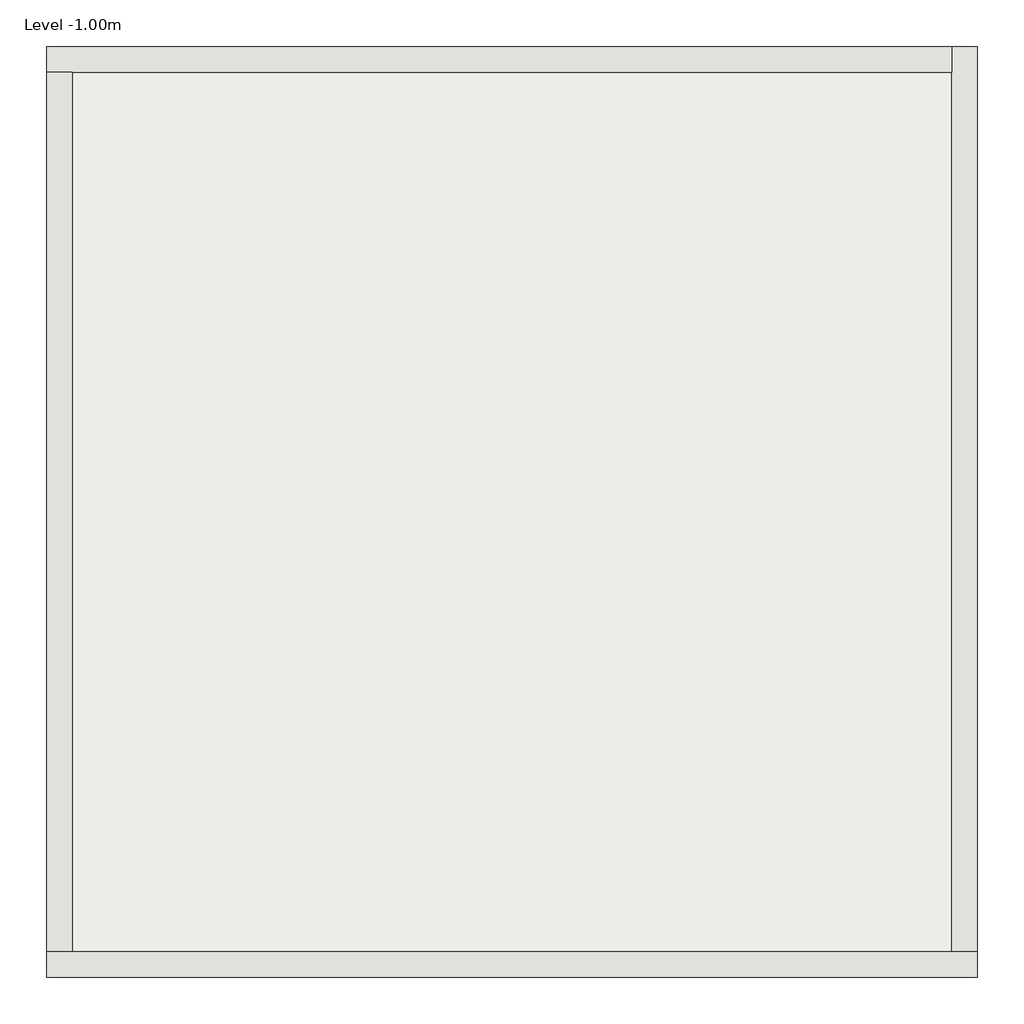
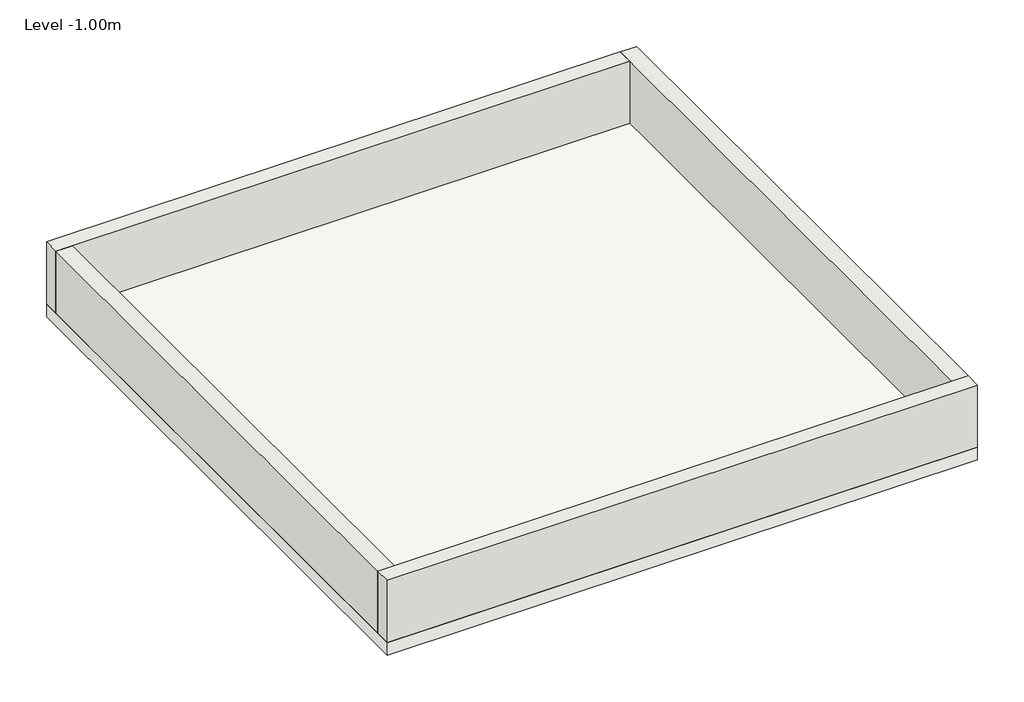
# One storey: 4 walls, 1 slab.
"""IFC4 building model written with IfcOpenShell, lengths in millimetres."""

from ifc_helpers import new_model, si_unit, frame, origin, place, context, project, spatial, polyline, outline, extrude, faceted_brep, element, save

model = new_model("IFC4")

# Units and contexts
model_context = context("Model", 3, world=origin())
ifc_project = project(units=[si_unit("LENGTHUNIT", "METRE", prefix="MILLI")], contexts=[model_context])

# Site, building, storey
site = spatial("IfcSite", under=ifc_project)
building = spatial("IfcBuilding", under=site)
storey = spatial("IfcBuildingStorey", under=building, Name="Level -1.00m", Elevation=-1000.0)

# Slab
placement = place(None, origin())
element("IfcSlab", 1, ObjectType="SOL CAM SANIT", at=placement, inside=storey, context=model_context, shape_type="SweptSolid", body=[
    extrude(outline(polyline([(0.0, 7999.99416), (9000.000032, 7999.99416), (9000.000032, -1000.005872), (0.0, -1000.005872), (0.0, 7999.99416)])), frame((0.0, 0.0, -1202.9999956), z_axis=(0.0, 0.0, 1.0), x_axis=(1.0, 0.0, 0.0)), (0.0, 0.0, 1.0), 202.9999956),
])

# Walls
element("IfcWall", 2, ObjectType="MURO CAM SANIT", at=placement, inside=storey, context=model_context, shape_type="Brep", body=[
    faceted_brep([(0.0, -1000.005872, -1000.0), (9000.000032, -1000.005872, -1000.0), (9000.000032, -1000.005872, -0.01216), (0.0, -1000.005872, -0.01216), (0.0, -751.005864, -1000.0), (0.0, -751.005864, -0.01216), (249.000008, -751.005864, -0.01216), (8751.000024, -751.005864, -0.01216), (9000.000032, -751.005864, -0.01216), (9000.000032, -751.005864, -1000.0), (8751.000024, -751.005864, -1000.0), (249.000008, -751.005864, -1000.0)], [[[0, 1, 2, 3]], [[4, 5, 6, 7, 8, 9, 10, 11]], [[1, 0, 4, 11, 10, 9]], [[3, 2, 8, 7, 6, 5]], [[2, 1, 9, 8]], [[0, 3, 5, 4]]]),
])
element("IfcWall", 3, ObjectType="MURO CAM SANIT", at=placement, inside=storey, context=model_context, shape_type="Brep", body=[
    faceted_brep([(9000.000032, -751.005864, -1000.0), (9000.000032, 7999.99416, -1000.0), (9000.000032, 7999.99416, -0.01216), (9000.000032, -751.005864, -0.01216), (8751.000024, -751.005864, -1000.0), (8751.000024, -751.005864, -0.01216), (8751.000024, 7750.994152, -0.01216), (8751.000024, 7999.99416, -0.01216), (8751.000024, 7999.99416, -1000.0), (8751.000024, 7750.994152, -1000.0)], [[[0, 1, 2, 3]], [[4, 5, 6, 7, 8, 9]], [[1, 0, 4, 9, 8]], [[3, 2, 7, 6, 5]], [[2, 1, 8, 7]], [[0, 3, 5, 4]]]),
])
element("IfcWall", 4, ObjectType="MURO CAM SANIT", at=placement, inside=storey, context=model_context, shape_type="Brep", body=[
    faceted_brep([(8751.000024, 7999.99416, -1000.0), (0.0, 7999.99416, -1000.0), (0.0, 7999.99416, -0.01216), (8751.000024, 7999.99416, -0.01216), (8751.000024, 7750.994152, -1000.0), (8751.000024, 7750.994152, -0.01216), (249.000008, 7750.994152, -0.01216), (0.0, 7750.994152, -0.01216), (0.0, 7750.994152, -1000.0), (249.000008, 7750.994152, -1000.0)], [[[0, 1, 2, 3]], [[4, 5, 6, 7, 8, 9]], [[1, 0, 4, 9, 8]], [[3, 2, 7, 6, 5]], [[2, 1, 8, 7]], [[0, 3, 5, 4]]]),
])
element("IfcWall", 5, ObjectType="MURO CAM SANIT", at=placement, inside=storey, context=model_context, shape_type="Brep", body=[
    faceted_brep([(0.0, 7750.994152, -1000.0), (0.0, -751.005864, -1000.0), (0.0, -751.005864, -0.01216), (0.0, 7499.994144, -0.01216), (0.0, 7750.994152, -0.01216), (249.000008, 7750.994152, -1000.0), (249.000008, 7750.994152, -0.01216), (249.000008, -751.005864, -0.01216), (249.000008, -751.005864, -1000.0)], [[[0, 1, 2, 3, 4]], [[5, 6, 7, 8]], [[1, 0, 5, 8]], [[4, 3, 2, 7, 6]], [[2, 1, 8, 7]], [[0, 4, 6, 5]]]),
])

save(model, "model.ifc")

# Revit data of these elements
# Project information
#   Organization Name = "Organization Name"
#   Organization Description = "Organization Description"
#   Building Name = "Building Name"
#   Project Issue Date = "Issue Date"
#   Project Status = "Project Status"
#   Client Name = "Client Name"
#   Project Address = "Enter address here\nAddress Line 2"
#   Project Name = "Project Name"
#   Project Number = "Project Number"
# Type "SOL CAM SANIT"
#   Layers, outside or top first: 0.080 m "Hormigón en masa d entre 2000 y 2300" (function 1); 0.003 m "Cloruro de polivinilo (PVC)" (function 1); 0.120 m "Arena y grava (d entre 1700 y 2200)" (function 1)
# Type "MURO CAM SANIT"
#   Description = "Metal Studs with Brick over sheathing on exterior and Gypsum Wall Board (GWB) on interior, Exterior Function"
#   Assembly Code = "B2010158"
#   Type Mark = "W10"
#   Layers, outside or top first: 0.009 m no material (function 1); 0.240 m no material (function 1)
# Element 1 (IfcSlab, "SOL CAM SANIT")
#   Height Offset From Level = 0.000 m
#   Phase Created = New Construction
#   Materials on its faces: "Arena y grava (d entre 1700 y 2200)", "Hormigón en masa d entre 2000 y 2300"
# Elements 2, 3, 4, 5 (IfcWall, "MURO CAM SANIT")
#   Comments = "BEM_GROUND_COUPLED"
#   Top Offset = 0.000 m
#   Base Offset = 0.000 m
#   Unconnected Height = 0.999988 m
#   wall height = 0.999988 m
#   Phase Created = New Construction
#   Base Constraint = Level -1.00m
#   Materials on its faces: "Default Wall"
# Materials
#   "Hormigón en masa d entre 2000 y 2300": class "Unassigned", colour RGB 0 0 0, transparency 0
#   "Cloruro de polivinilo (PVC)": class "Unassigned", colour RGB 0 0 0, transparency 0
#   "Arena y grava (d entre 1700 y 2200)": class "Unassigned", colour RGB 0 0 0, transparency 0
#   "Default Wall": class "Miscellaneous", colour RGB 192 192 192, transparency 0, Cost = 0
